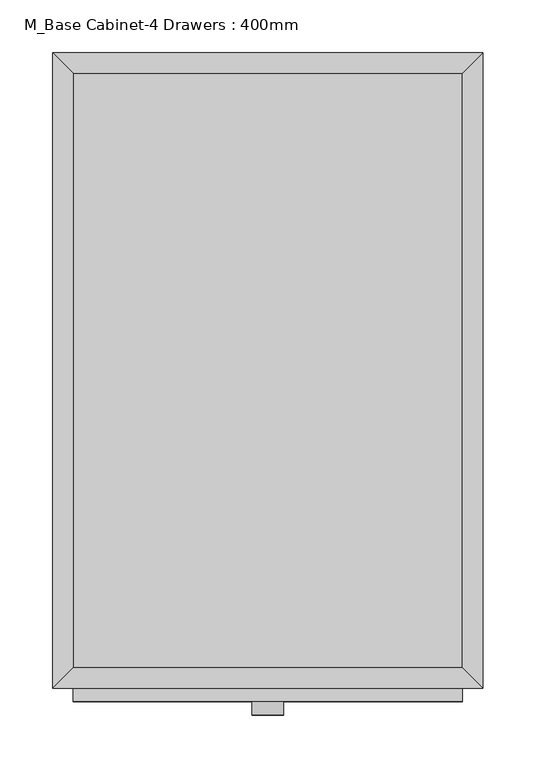
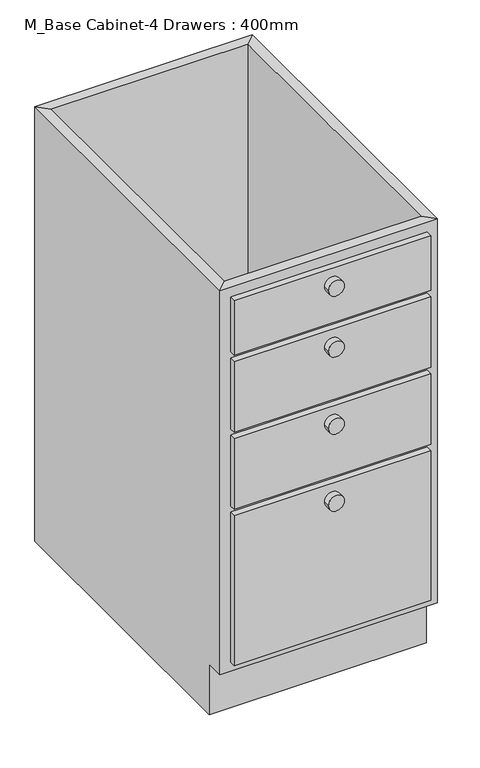
"""IFC4 building model written with IfcOpenShell, lengths in millimetres: furniture geometry, M_Base Cabinet-4 Drawers : 400mm."""

from ifc_helpers import new_model, si_unit, point, frame, frame_2d, origin, place, context, project, spatial, polyline, circle_curve, trimmed, segment, composite_curve, outline, extrude, faceted_brep, source, transform, mapped, element, save


def m_base_cabinet_4_drawers_400mm_697f473e(model_context):
    return source(origin(), model_context, "Body", "SolidModel", [
        faceted_brep([(202.8877049, -580.95, 860.0), (202.8877049, -580.95, 100.0), (-165.4122951, -580.95, 100.0), (-165.4122951, -580.95, 860.0), (-184.4622951, -600.0, 860.0), (221.9377049, -600.0, 860.0), (-184.4622951, -600.0, 100.0), (221.9377049, -600.0, 100.0), (-165.4122951, -565.0, 100.0), (-165.4122951, -19.05, 100.0), (-165.4122951, -19.05, 860.0), (-184.4622951, 0.0, 860.0), (-184.4622951, 0.0, 0.0), (-184.4622951, -565.0, 0.0), (-184.4622951, -565.0, 100.0), (202.8877049, -19.05, 100.0), (202.8877049, -19.05, 860.0), (221.9377049, 0.0, 860.0), (221.9377049, 0.0, 0.0), (202.8877049, -565.0, 100.0), (221.9377049, -565.0, 100.0), (221.9377049, -565.0, 0.0)], [[[0, 1, 2, 3]], [[0, 3, 4, 5]], [[5, 4, 6, 7]], [[2, 1, 7, 6]], [[3, 2, 8, 9, 10]], [[4, 3, 10, 11]], [[6, 4, 11, 12, 13, 14]], [[2, 6, 14, 8]], [[10, 9, 15, 16]], [[11, 10, 16, 17]], [[12, 11, 17, 18]], [[1, 0, 16, 15, 19]], [[0, 5, 17, 16]], [[5, 7, 20, 21, 18, 17]], [[7, 1, 19, 20]], [[8, 19, 15, 9]], [[18, 21, 13, 12]], [[13, 21, 20, 19, 8, 14]]]),
        extrude(outline(composite_curve([segment(trimmed(circle_curve(frame_2d((809.2, 18.7377049)), 15.0), [point((809.2, 3.7377049))], [point((809.2, 33.7377049))], False, "CARTESIAN"), True, "CONTINUOUS"), segment(trimmed(circle_curve(frame_2d((809.2, 18.7377049)), 15.0), [point((809.2, 33.7377049))], [point((809.2, 3.7377049))], False, "CARTESIAN"), True, "CONTINUOUS")], self_intersect=False)), frame((0.0, -625.4, 0.0), z_axis=(0.0, 1.0, 0.0), x_axis=(0.0, 0.0, 1.0)), (0.0, 0.0, 1.0), 12.7),
        extrude(outline(composite_curve([segment(trimmed(circle_curve(frame_2d((688.55, 18.7377049)), 15.0), [point((688.55, 3.7377049))], [point((688.55, 33.7377049))], False, "CARTESIAN"), True, "CONTINUOUS"), segment(trimmed(circle_curve(frame_2d((688.55, 18.7377049)), 15.0), [point((688.55, 33.7377049))], [point((688.55, 3.7377049))], False, "CARTESIAN"), True, "CONTINUOUS")], self_intersect=False)), frame((0.0, -625.4, 0.0), z_axis=(0.0, 1.0, 0.0), x_axis=(0.0, 0.0, 1.0)), (0.0, 0.0, 1.0), 12.7),
        extrude(outline(composite_curve([segment(trimmed(circle_curve(frame_2d((536.15, 18.7377049)), 15.0), [point((536.15, 3.7377049))], [point((536.15, 33.7377049))], False, "CARTESIAN"), True, "CONTINUOUS"), segment(trimmed(circle_curve(frame_2d((536.15, 18.7377049)), 15.0), [point((536.15, 33.7377049))], [point((536.15, 3.7377049))], False, "CARTESIAN"), True, "CONTINUOUS")], self_intersect=False)), frame((0.0, -625.4, 0.0), z_axis=(0.0, 1.0, 0.0), x_axis=(0.0, 0.0, 1.0)), (0.0, 0.0, 1.0), 12.7),
        extrude(outline(composite_curve([segment(trimmed(circle_curve(frame_2d((383.75, 18.7377049)), 15.0), [point((383.75, 3.7377049))], [point((383.75, 33.7377049))], False, "CARTESIAN"), True, "CONTINUOUS"), segment(trimmed(circle_curve(frame_2d((383.75, 18.7377049)), 15.0), [point((383.75, 33.7377049))], [point((383.75, 3.7377049))], False, "CARTESIAN"), True, "CONTINUOUS")], self_intersect=False)), frame((0.0, -625.4, 0.0), z_axis=(0.0, 1.0, 0.0), x_axis=(0.0, 0.0, 1.0)), (0.0, 0.0, 1.0), 12.7),
        extrude(outline(polyline([(202.8877049, -612.7), (-165.4122951, -612.7), (-165.4122951, -600.0), (202.8877049, -600.0), (202.8877049, -612.7)])), frame((0.0, 0.0, 733.0), z_axis=(0.0, 0.0, 1.0), x_axis=(1.0, 0.0, 0.0)), (0.0, 0.0, 1.0), 107.95),
        extrude(outline(polyline([(202.8877049, -612.7), (-165.4122951, -612.7), (-165.4122951, -600.0), (202.8877049, -600.0), (202.8877049, -612.7)])), frame((0.0, 0.0, 580.6), z_axis=(0.0, 0.0, 1.0), x_axis=(1.0, 0.0, 0.0)), (0.0, 0.0, 1.0), 139.7),
        extrude(outline(polyline([(202.8877049, -612.7), (-165.4122951, -612.7), (-165.4122951, -600.0), (202.8877049, -600.0), (202.8877049, -612.7)])), frame((0.0, 0.0, 428.2), z_axis=(0.0, 0.0, 1.0), x_axis=(1.0, 0.0, 0.0)), (0.0, 0.0, 1.0), 139.7),
        extrude(outline(polyline([(202.8877049, -612.7), (-165.4122951, -612.7), (-165.4122951, -600.0), (202.8877049, -600.0), (202.8877049, -612.7)])), frame((0.0, 0.0, 119.05), z_axis=(0.0, 0.0, 1.0), x_axis=(1.0, 0.0, 0.0)), (0.0, 0.0, 1.0), 296.45),
        extrude(outline(polyline([(202.8877049, -19.05), (202.8877049, -580.95), (-165.4122951, -580.95), (-165.4122951, -19.05), (202.8877049, -19.05)])), frame((0.0, 0.0, 100.0), z_axis=(0.0, 0.0, 1.0), x_axis=(1.0, 0.0, 0.0)), (0.0, 0.0, 1.0), 19.05),
    ])


if __name__ == "__main__":
    model = new_model("IFC4")
    model_context = context("Model", 3, world=origin())
    ifc_project = project(units=[si_unit("LENGTHUNIT", "METRE", prefix="MILLI")], contexts=[model_context])
    site = spatial("IfcSite", under=ifc_project)
    building = spatial("IfcBuilding", under=site)
    placement = place(None, origin())
    m_base_cabinet_4_drawers_400mm_shape = m_base_cabinet_4_drawers_400mm_697f473e(model_context)
    element("IfcFurniture", 1, ObjectType="M_Base Cabinet-4 Drawers : 400mm", at=placement, inside=building, context=model_context, shape_type="MappedRepresentation", body=[
        mapped(m_base_cabinet_4_drawers_400mm_shape, transform((0.0, 0.0, 0.0), x_axis=(1.0, 0.0, 0.0), y_axis=(0.0, 1.0, 0.0), z_axis=(0.0, 0.0, 1.0))),
    ])
    save(model, "model.ifc")

# Revit data of these elements
# Type "M_Base Cabinet-4 Drawers : 400mm"
#   Depth = 1' - 11.62205"
#   Height = 2' - 9.85827"
#   Plinth Depth = 0' - 1.37795"
#   Plinth Height = 0' - 3.93701"
#   Width = 1' - 4"
#   Cabinet Material = Base cabinet 2120100 Aspekt - 83012120100 - White
#   Door/Drawer Material = Base cabinet 2120100 Aspekt - 83012120100 - White
#   Handle Material = Cabinets - Handles
#   Default Elevation = 0
# Element 1 (IfcFurniture, "M_Base Cabinet-4 Drawers : 400mm")
#   Materials on its faces: "Base cabinet 2120100 Aspekt - 83012120100 - White", "Cabinets - Handles"
# Materials
#   "Base cabinet 2120100 Aspekt - 83012120100 - White": class "Miscellaneous", colour RGB 255 255 255, transparency 0, Manufacturer = "Marbodal", URL = "http://www.marbodal.se", Cost = 0
#   "Cabinets - Handles": class "Metal", colour RGB 57 57 57, transparency 0
